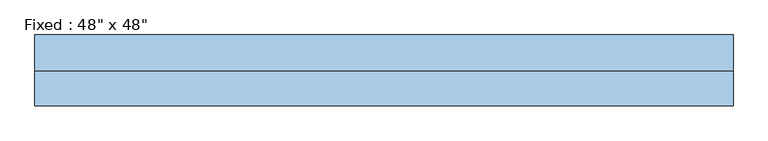
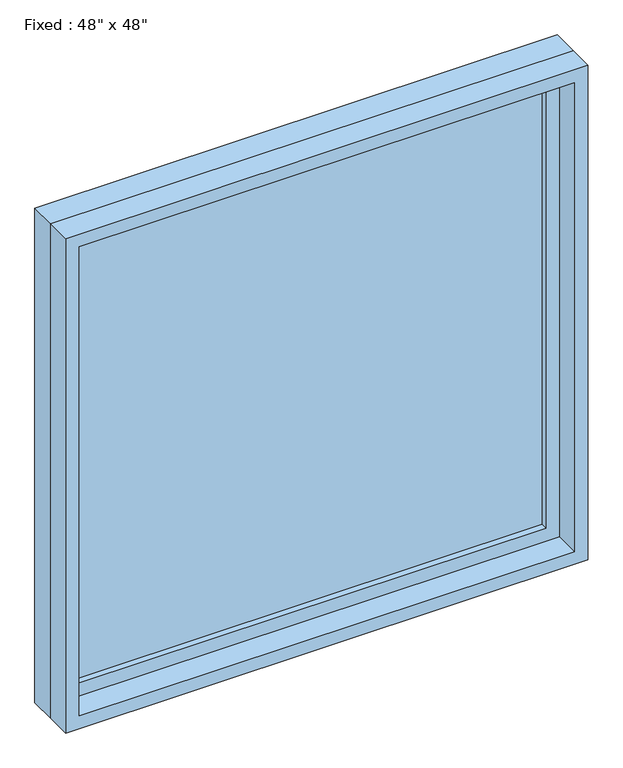
"""IFC4 building model written with IfcOpenShell, lengths in millimetres: window geometry."""

import ifcopenshell
import ifcopenshell.guid

model = None  # the IFC model being written
_history = None  # IfcOwnerHistory: only IFC2X3 demands one
_inside = {}  # id of a spatial element -> (the spatial element, [elements in it])
_under = {}  # id of a project, library or spatial element -> (it, [spatial elements below it])
_declared = {}  # id of a project -> (the project, [libraries it declares])
_typed = {}  # id of a type object -> (the type object, [elements of that type])
_made_of = {}  # id of a material, layer set ... -> (it, [elements and type objects made of it])


def new_model(schema):
    """Start an empty IFC model of exactly this schema.

    Asked for "IFC4X3", IfcOpenShell would pick the latest addendum, in which some entities
    have other attributes; the version numbers below select the first issue.
    IFC2X3 requires an IfcOwnerHistory on every rooted entity: one is made here for all.
    """
    global model, _history
    if schema == "IFC4X3":
        model = ifcopenshell.file(schema_version=(4, 3, 0, 0))
    else:
        model = ifcopenshell.file(schema=schema)
    _inside.clear()
    _under.clear()
    _declared.clear()
    _typed.clear()
    _made_of.clear()
    _history = None
    if model.schema == "IFC2X3":
        org = make("IfcOrganization", Name="unknown")
        user = make(
            "IfcPersonAndOrganization",
            ThePerson=make("IfcPerson", FamilyName="unknown"),
            TheOrganization=org,
        )
        app = make(
            "IfcApplication",
            ApplicationDeveloper=org,
            Version="unknown",
            ApplicationFullName="unknown",
            ApplicationIdentifier="unknown",
        )
        _history = make(
            "IfcOwnerHistory",
            OwningUser=user,
            OwningApplication=app,
            ChangeAction="ADDED",
            CreationDate=0,
        )
    return model


def make(cls, **values):
    """One entity of the class cls with the attributes given. An attribute that is None is left unset."""
    return model.create_entity(
        cls, **{name: value for name, value in values.items() if value is not None}
    )


def rooted(cls, **values):
    """An entity with a GlobalId (a new one), such as an element, a storey or a relation."""
    return make(cls, GlobalId=ifcopenshell.guid.new(), OwnerHistory=_history, **values)


def si_unit(unit_type, name, prefix=None):
    """IfcSIUnit, for example si_unit("LENGTHUNIT", "METRE", prefix="MILLI")."""
    return make("IfcSIUnit", UnitType=unit_type, Prefix=prefix, Name=name)


def assignment(units):
    """IfcUnitAssignment: the units of a project."""
    return None if units is None else make("IfcUnitAssignment", Units=units)


def point(xyz):
    """IfcCartesianPoint."""
    return None if xyz is None else make("IfcCartesianPoint", Coordinates=xyz)


def direction(xyz):
    """IfcDirection."""
    return None if xyz is None else make("IfcDirection", DirectionRatios=xyz)


def frame(location, z_axis=None, x_axis=None):
    """IfcAxis2Placement3D, a coordinate frame: its origin and axes. An axis left out is left unset."""
    return make(
        "IfcAxis2Placement3D",
        Location=point(location),
        Axis=direction(z_axis),
        RefDirection=direction(x_axis),
    )


def origin():
    """The frame at (0, 0, 0) with its axes left unset."""
    return frame((0.0, 0.0, 0.0))


def place(relative_to, where):
    """IfcLocalPlacement: puts the frame where relative to a parent placement (None: the world)."""
    return make(
        "IfcLocalPlacement", PlacementRelTo=relative_to, RelativePlacement=where
    )


def context(
    kind, dimensions, precision=None, world=None, true_north=None, identifier=None
):
    """IfcGeometricRepresentationContext, for example the 3D "Model" context."""
    return make(
        "IfcGeometricRepresentationContext",
        ContextIdentifier=identifier,
        ContextType=kind,
        CoordinateSpaceDimension=dimensions,
        Precision=precision,
        WorldCoordinateSystem=world,
        TrueNorth=true_north,
    )


def project(units=None, contexts=None):
    """IfcProject with its units and contexts."""
    return rooted(
        "IfcProject",
        Name="project",
        RepresentationContexts=contexts,
        UnitsInContext=assignment(units),
    )


def spatial(cls, under=None, at=None, **own):
    """A site, building, storey or space (cls), placed at a placement, below another one or the project."""
    s = rooted(cls, ObjectPlacement=at, **own)
    if under is not None:
        _under.setdefault(under.id(), (under, []))[1].append(s)
    return s


def polyline(points):
    """IfcPolyline through the points."""
    return make("IfcPolyline", Points=[point(p) for p in points])


def outline(outer, holes=None, kind="AREA"):
    """IfcArbitraryClosedProfileDef: a profile drawn as a closed curve; with holes, ...WithVoids."""
    if holes is None:
        return make("IfcArbitraryClosedProfileDef", ProfileType=kind, OuterCurve=outer)
    return make(
        "IfcArbitraryProfileDefWithVoids",
        ProfileType=kind,
        OuterCurve=outer,
        InnerCurves=holes,
    )


def extrude(swept, where, along, depth):
    """IfcExtrudedAreaSolid: the profile swept, set in the frame where, extruded along a direction by depth."""
    return make(
        "IfcExtrudedAreaSolid",
        SweptArea=swept,
        Position=where,
        ExtrudedDirection=direction(along),
        Depth=depth,
    )


def shape(context_of_items, identifier, shape_type, items):
    """IfcShapeRepresentation: the items that make up one representation, for example the "Body"."""
    return make(
        "IfcShapeRepresentation",
        ContextOfItems=context_of_items,
        RepresentationIdentifier=identifier,
        RepresentationType=shape_type,
        Items=items,
    )


def source(mapping_origin, context_of_items, identifier, shape_type, items):
    """IfcRepresentationMap: a shape defined once, which mapped items show again and again."""
    return make(
        "IfcRepresentationMap",
        MappingOrigin=mapping_origin,
        MappedRepresentation=shape(context_of_items, identifier, shape_type, items),
    )


def transform(
    local_origin,
    x_axis=None,
    y_axis=None,
    z_axis=None,
    scale=None,
    scale2=None,
    scale3=None,
    uniform=True,
):
    """IfcCartesianTransformationOperator3D, or its non-uniform kind. x_axis, y_axis, z_axis: its Axis1, 2, 3."""
    if uniform:
        return make(
            "IfcCartesianTransformationOperator3D",
            Axis1=direction(x_axis),
            Axis2=direction(y_axis),
            LocalOrigin=point(local_origin),
            Scale=scale,
            Axis3=direction(z_axis),
        )
    return make(
        "IfcCartesianTransformationOperator3DnonUniform",
        Axis1=direction(x_axis),
        Axis2=direction(y_axis),
        LocalOrigin=point(local_origin),
        Scale=scale,
        Axis3=direction(z_axis),
        Scale2=scale2,
        Scale3=scale3,
    )


def mapped(mapping_source, mapping_target):
    """IfcMappedItem: shows the shape of a source again, moved by a transform."""
    return make(
        "IfcMappedItem", MappingSource=mapping_source, MappingTarget=mapping_target
    )


def made_of(thing, what):
    """Note that an element or type object is made of a material, layer set ...; save() writes the relation."""
    if what is not None:
        _made_of.setdefault(what.id(), (what, []))[1].append(thing)
    return thing


def element(
    cls,
    number,
    at=None,
    inside=None,
    cuts=None,
    type_object=None,
    material=None,
    context=None,
    identifier="Body",
    shape_type=None,
    held_by="IfcProductDefinitionShape",
    body=None,
    shapes=None,
    **own,
):
    """One element of the class cls, such as IfcWall. Its Tag is "e" and its number.

    at: its placement. inside: the storey or other place that contains it. cuts: it is an
    opening in that element (IfcRelVoidsElement). A single representation is given by context,
    identifier, shape_type and body (its items); several are given by shapes. held_by: the class
    of the entity that holds the representations. save() writes the other relations.
    """
    e = rooted(cls, Tag="e%d" % number, ObjectPlacement=at, **own)
    if body is not None:
        shapes = [shape(context, identifier, shape_type, body)]
    if shapes is not None:
        e.Representation = make(held_by, Representations=shapes)
    if inside is not None:
        _inside.setdefault(inside.id(), (inside, []))[1].append(e)
    if cuts is not None:
        rooted(
            "IfcRelVoidsElement", RelatingBuildingElement=cuts, RelatedOpeningElement=e
        )
    if type_object is not None:
        _typed.setdefault(type_object.id(), (type_object, []))[1].append(e)
    return made_of(e, material)


def aggregate(whole, parts):
    """IfcRelAggregates: a whole, such as a stair, and the parts it consists of."""
    return rooted("IfcRelAggregates", RelatingObject=whole, RelatedObjects=parts)


def save(model, path):
    """Write the relations noted so far, then the file.

    IfcRelAggregates (storeys below a building ...), IfcRelContainedInSpatialStructure (elements
    in a storey), IfcRelDefinesByType, IfcRelAssociatesMaterial and IfcRelDeclares: one each for
    every whole, place, type object, material and project.
    """
    for whole, parts in _under.values():
        aggregate(whole, parts)
    for where, things in _inside.values():
        rooted(
            "IfcRelContainedInSpatialStructure",
            RelatedElements=things,
            RelatingStructure=where,
        )
    for kind, things in _typed.values():
        rooted("IfcRelDefinesByType", RelatedObjects=things, RelatingType=kind)
    for what, things in _made_of.values():
        rooted("IfcRelAssociatesMaterial", RelatedObjects=things, RelatingMaterial=what)
    for by, libraries in _declared.values():
        rooted("IfcRelDeclares", RelatingContext=by, RelatedDefinitions=libraries)
    model.write(path)


def window_0af993c7(model_context):
    return source(origin(), model_context, "Body", "SweptSolid", [
        extrude(outline(polyline([(508.0, 14.2875), (-584.2, 14.2875), (-584.2, 26.9875), (508.0, 26.9875), (508.0, 14.2875)])), frame((0.0, 0.0, 977.9), z_axis=(0.0, 0.0, 1.0), x_axis=(1.0, 0.0, 0.0)), (0.0, 0.0, 1.0), 1092.2),
        extrude(outline(polyline([(2114.55, -628.65), (933.45, -628.65), (933.45, 552.45), (2114.55, 552.45), (2114.55, -628.65)]), holes=[polyline([(2070.1, -584.2), (2070.1, 508.0), (977.9, 508.0), (977.9, -584.2), (2070.1, -584.2)])]), frame((0.0, -1.5875, 0.0), z_axis=(0.0, 1.0, 0.0), x_axis=(0.0, 0.0, 1.0)), (0.0, 0.0, 1.0), 44.45),
        extrude(outline(polyline([(2133.6, -647.7), (914.4, -647.7), (914.4, 571.5), (2133.6, 571.5), (2133.6, -647.7)]), holes=[polyline([(2101.85, -615.95), (2101.85, 539.75), (946.15, 539.75), (946.15, -615.95), (2101.85, -615.95)])]), frame((0.0, -61.9125, 0.0), z_axis=(0.0, 1.0, 0.0), x_axis=(0.0, 0.0, 1.0)), (0.0, 0.0, 1.0), 60.325),
        extrude(outline(polyline([(2133.6, 571.5), (2133.6, -647.7), (914.4, -647.7), (914.4, 571.5), (2133.6, 571.5)]), holes=[polyline([(2114.55, 552.45), (933.45, 552.45), (933.45, -628.65), (2114.55, -628.65), (2114.55, 552.45)])]), frame((0.0, -1.5875, 0.0), z_axis=(0.0, 1.0, 0.0), x_axis=(0.0, 0.0, 1.0)), (0.0, 0.0, 1.0), 63.5),
    ])


if __name__ == "__main__":
    model = new_model("IFC4")
    model_context = context("Model", 3, world=origin())
    ifc_project = project(units=[si_unit("LENGTHUNIT", "METRE", prefix="MILLI")], contexts=[model_context])
    site = spatial("IfcSite", under=ifc_project)
    building = spatial("IfcBuilding", under=site)
    placement = place(None, origin())
    window_shape = window_0af993c7(model_context)
    element("IfcWindow", 1, ObjectType="Fixed : 48\" x 48\"", at=placement, inside=building, context=model_context, shape_type="MappedRepresentation", body=[
        mapped(window_shape, transform((0.0, 0.0, 0.0), x_axis=(1.0, 0.0, 0.0), y_axis=(0.0, 1.0, 0.0), z_axis=(0.0, 0.0, 1.0))),
    ])
    save(model, "model.ifc")

# Revit data of these elements
# Project information
#   Room Abbreviation = "NMGS1"
#   Room Description = "Scanning Room, Nuclear Medicine (NMGS1)"
#   Sheets - Total = "6"
#   Project Issue Date = "Issue Date"
#   Project Status = "Project Status"
#   Client Name = "Owner"
#   Project Address = "Enter address here"
#   Project Name = "Project Name"
#   Project Number = "Project Number"
#   Publication Date = "30-Jan-15"
# Type "Fixed : 48\" x 48\""
#   Type Mark = "12"
#   Assembly Code = "B2020100"
#   Height = 4' - 0"
#   Default Sill Height = 3' - 0"
#   Width = 4' - 0"
#   Window Inset = 0' - 0 3/4"
#   Glass Pane Material = Glass
#   Sash Material = Sash
#   Wall Closure = (empty or 0)
# Element 1 (IfcWindow, "Fixed : 48\" x 48\"")
#   Materials on its faces: "Sash", "Glass"
# Materials
#   "Glass": class "Glass", colour RGB 0 128 192, transparency 0.75
#   "Sash": class "Wood", colour RGB 224 178 126, transparency 0
